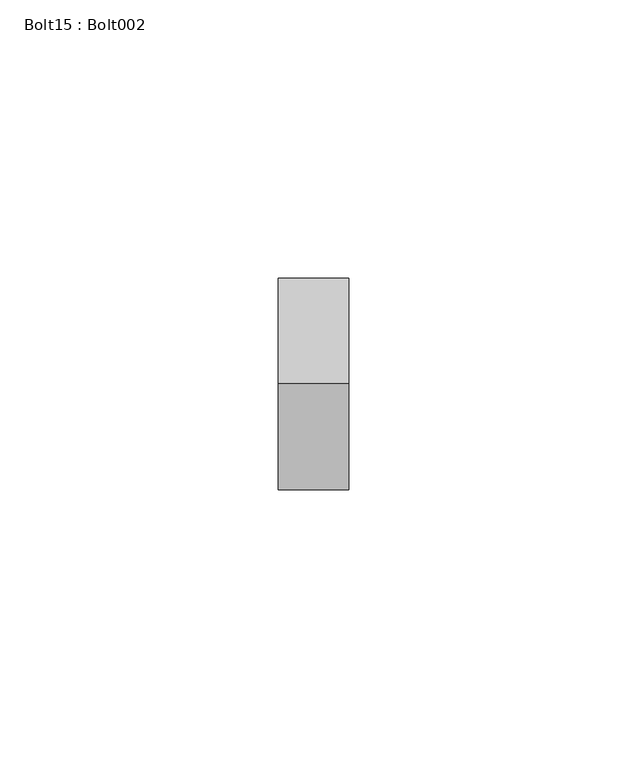
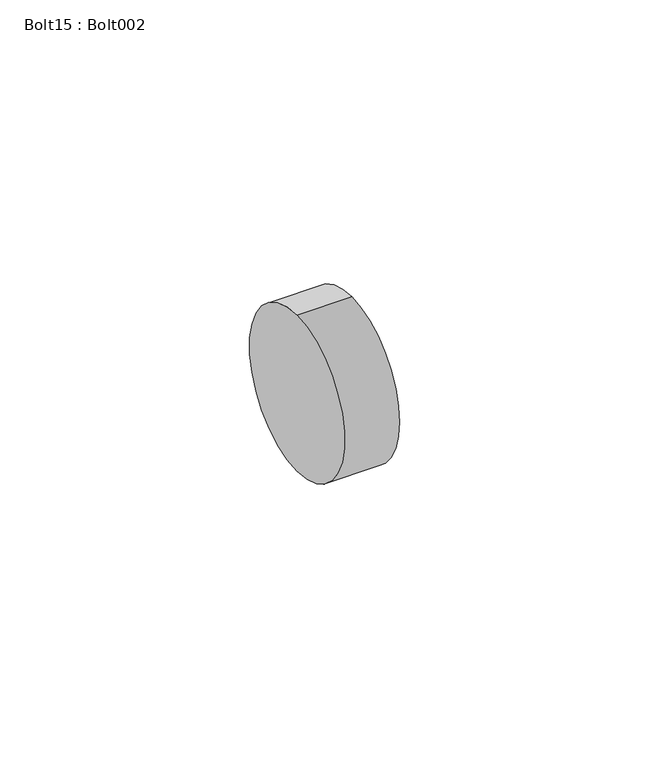
"""IFC4 building model written with IfcOpenShell, lengths in millimetres: proxy geometry, Bolt15 : Bolt002."""

from ifc_helpers import new_model, si_unit, point, frame, frame_2d, origin, place, context, project, spatial, circle_curve, trimmed, segment, composite_curve, outline, extrude, source, transform, mapped, element, save


def bolt15_bolt002_170dc097(model_context):
    return source(origin(), model_context, "Body", "SweptSolid", [
        extrude(outline(composite_curve([segment(trimmed(circle_curve(frame_2d((1896.5882072, 39910.0063132)), 19.05), [point((1896.5882072, 39929.0563132))], [point((1896.5882072, 39890.9563132))], False, "CARTESIAN"), True, "CONTINUOUS"), segment(trimmed(circle_curve(frame_2d((1896.5882072, 39910.0063132)), 19.05), [point((1896.5882072, 39890.9563132))], [point((1896.5882072, 39929.0563132))], False, "CARTESIAN"), True, "CONTINUOUS")], self_intersect=False)), frame((10297.8384869, 0.0, 0.0), z_axis=(1.0, 0.0, 0.0), x_axis=(0.0, 1.0, 0.0)), (0.0, 0.0, 1.0), 12.7),
    ])


if __name__ == "__main__":
    model = new_model("IFC4")
    model_context = context("Model", 3, world=origin())
    ifc_project = project(units=[si_unit("LENGTHUNIT", "METRE", prefix="MILLI")], contexts=[model_context])
    site = spatial("IfcSite", under=ifc_project)
    building = spatial("IfcBuilding", under=site)
    placement = place(None, origin())
    bolt15_bolt002_shape = bolt15_bolt002_170dc097(model_context)
    element("IfcBuildingElementProxy", 1, Name="Bolt15 : Bolt002", ObjectType="Bolt15 : Bolt002", at=placement, inside=building, context=model_context, shape_type="MappedRepresentation", body=[
        mapped(bolt15_bolt002_shape, transform((0.0, 0.0, 0.0), x_axis=(1.0, 0.0, 0.0), y_axis=(0.0, 1.0, 0.0), z_axis=(0.0, 0.0, 1.0))),
    ])
    save(model, "model.ifc")

# Revit data of these elements
# Type "Bolt15 : Bolt002"
#   NameOverride = "Bolt002"
# Element 1 (IfcBuildingElementProxy, "Bolt15 : Bolt002")
#   Materials on its faces: "TUBE STEEL STRINGER WELDED TO ANCHORED STEEL PLATE - SEE STRUCT DWGS"
# Materials
#   "TUBE STEEL STRINGER WELDED TO ANCHORED STEEL PLATE - SEE STRUCT DWGS": class "Unassigned", colour RGB 128 128 128, transparency 0, Cost = 0
